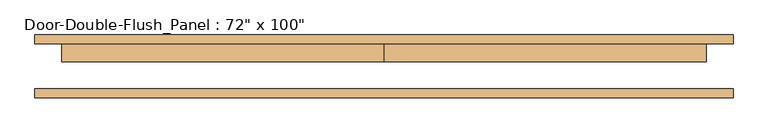
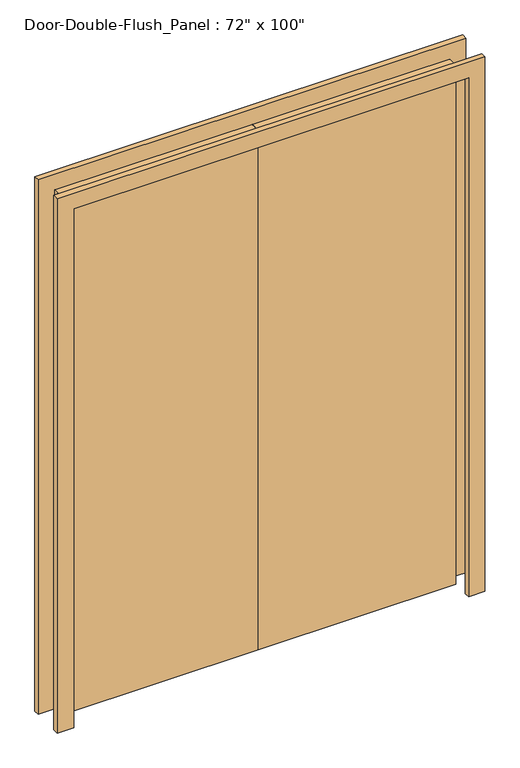
"""IFC4 building model written with IfcOpenShell, lengths in millimetres: door geometry."""

from ifc_helpers import new_model, si_unit, frame, origin, origin_with_axes, place, context, project, spatial, polyline, outline, extrude, source, transform, mapped, element, save


def door_4d6d2880(model_context):
    return source(origin(), model_context, "Body", "SweptSolid", [
        extrude(outline(polyline([(2540.0, -914.4), (2540.0, 914.4), (0.0, 914.4), (0.0, 990.6), (2616.2, 990.6), (2616.2, -990.6), (0.0, -990.6), (0.0, -914.4), (2540.0, -914.4)])), frame((0.0, -88.9, 0.0), z_axis=(0.0, 1.0, 0.0), x_axis=(0.0, 0.0, 1.0)), (0.0, 0.0, 1.0), 25.4),
        extrude(outline(polyline([(2540.0, -914.4), (2540.0, 914.4), (0.0, 914.4), (0.0, 990.6), (2616.2, 990.6), (2616.2, -990.6), (0.0, -990.6), (0.0, -914.4), (2540.0, -914.4)])), frame((0.0, 63.5, 0.0), z_axis=(0.0, 1.0, 0.0), x_axis=(0.0, 0.0, 1.0)), (0.0, 0.0, 1.0), 25.4),
        extrude(outline(polyline([(0.0, 63.5), (914.4, 63.5), (914.4, 12.7), (0.0, 12.7), (0.0, 63.5)])), origin_with_axes(), (0.0, 0.0, 1.0), 2540.0),
        extrude(outline(polyline([(-914.4, 63.5), (0.0, 63.5), (0.0, 12.7), (-914.4, 12.7), (-914.4, 63.5)])), origin_with_axes(), (0.0, 0.0, 1.0), 2540.0),
    ])


if __name__ == "__main__":
    model = new_model("IFC4")
    model_context = context("Model", 3, world=origin())
    ifc_project = project(units=[si_unit("LENGTHUNIT", "METRE", prefix="MILLI")], contexts=[model_context])
    site = spatial("IfcSite", under=ifc_project)
    building = spatial("IfcBuilding", under=site)
    placement = place(None, origin())
    door_shape = door_4d6d2880(model_context)
    element("IfcDoor", 1, ObjectType="Door-Double-Flush_Panel : 72\" x 100\"", at=placement, inside=building, context=model_context, shape_type="MappedRepresentation", body=[
        mapped(door_shape, transform((0.0, 0.0, 0.0), x_axis=(1.0, 0.0, 0.0), y_axis=(0.0, 1.0, 0.0), z_axis=(0.0, 0.0, 1.0))),
    ])
    save(model, "model.ifc")

# Revit data of these elements
# Type "Door-Double-Flush_Panel : 72\" x 100\""
#   Type Mark = "9"
#   Construction Type Id = "DOOR"
#   Assembly Code = "C1020"
#   Analytic Construction = "Wooden"
#   Thickness = 0' - 2"
#   Thermal Resistance (R) = 0.455703 (m²·K)/W
#   Swing Angle [instance default] = 90.00°
#   Panel Width = 3' - 0"
#   Heat Transfer Coefficient (U) = 2.19465 W/(m²·K)
#   Height = 8' - 4"
#   Trim Projection Ext = 0' - 1"
#   Trim Projection Int = 0' - 1"
#   Trim Width = 0' - 3"
#   Width = 6' - 0"
#   Panel Material = WOOD VENEER PANELING (MATCH WOOD AT CLOSET DOORS)
#   Trim Material = ALUM
#   Visual Light Transmittance = 0
#   Solar Heat Gain Coefficient = 0
#   Function = (empty or 0)
#   Wall Closure = (empty or 0)
# Element 1 (IfcDoor, "Door-Double-Flush_Panel : 72\" x 100\"")
#   Materials on its faces: "ALUM", "WOOD VENEER PANELING (MATCH WOOD AT CLOSET DOORS)"
# Materials
#   "WOOD VENEER PANELING (MATCH WOOD AT CLOSET DOORS)": class "Wood", colour RGB 255 253 232, transparency 0, Cost = 0
#   "ALUM": class "Generic", colour RGB 157 157 157, transparency 0, Cost = 0
